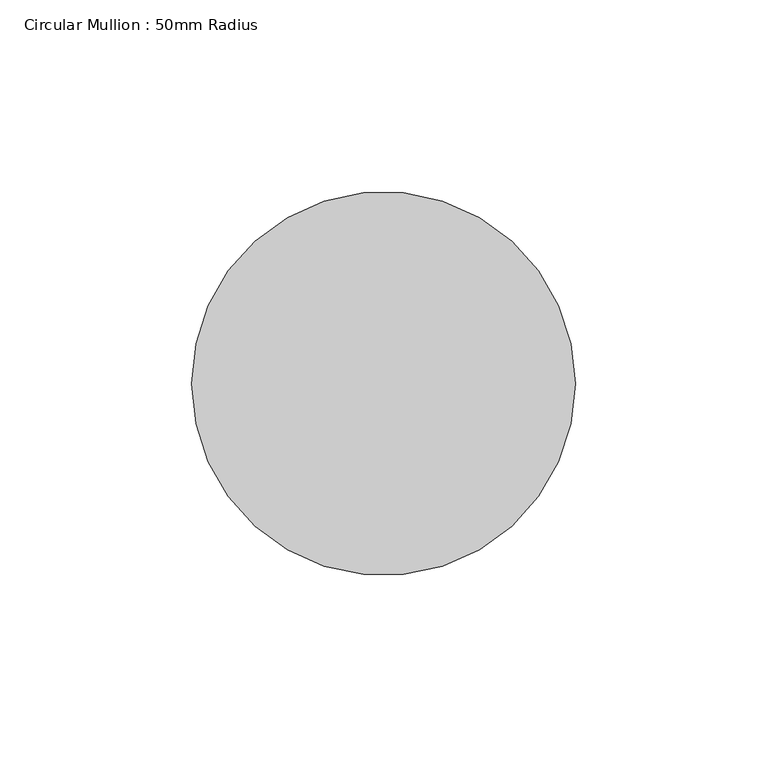
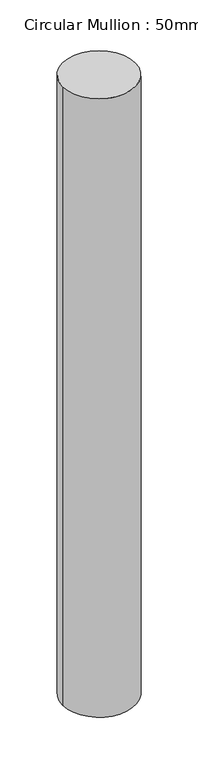
"""IFC4 building model written with IfcOpenShell, lengths in millimetres: member geometry, Circular Mullion : 50mm Radius."""

from ifc_helpers import new_model, si_unit, point, frame, origin, origin_2d, place, context, project, spatial, circle_curve, trimmed, segment, composite_curve, outline, extrude, source, transform, mapped, element, save


def circular_mullion_50mm_radius_7659f404(model_context):
    return source(origin(), model_context, "Body", "SweptSolid", [
        extrude(outline(composite_curve([segment(trimmed(circle_curve(origin_2d(), 50.0), [point((50.0, 0.0))], [point((-50.0, 0.0))], False, "CARTESIAN"), True, "CONTINUOUS"), segment(trimmed(circle_curve(origin_2d(), 50.0), [point((-50.0, 0.0))], [point((50.0, 0.0))], False, "CARTESIAN"), True, "CONTINUOUS")], self_intersect=False)), frame((0.0, 0.0, -900.5440201), z_axis=(0.0, 0.0, 1.0), x_axis=(1.0, 0.0, 0.0)), (0.0, 0.0, 1.0), 900.5440201),
    ])


if __name__ == "__main__":
    model = new_model("IFC4")
    model_context = context("Model", 3, world=origin())
    ifc_project = project(units=[si_unit("LENGTHUNIT", "METRE", prefix="MILLI")], contexts=[model_context])
    site = spatial("IfcSite", under=ifc_project)
    building = spatial("IfcBuilding", under=site)
    placement = place(None, origin())
    circular_mullion_50mm_radius_shape = circular_mullion_50mm_radius_7659f404(model_context)
    element("IfcMember", 1, ObjectType="Circular Mullion : 50mm Radius", at=placement, inside=building, context=model_context, shape_type="MappedRepresentation", body=[
        mapped(circular_mullion_50mm_radius_shape, transform((0.0, 0.0, 0.0), x_axis=(1.0, 0.0, 0.0), y_axis=(0.0, 1.0, 0.0), z_axis=(0.0, 0.0, 1.0))),
    ])
    save(model, "model.ifc")

# Revit data of these elements
# Type "Circular Mullion : 50mm Radius"
#   built-in parameter 1007350 = 0.164042 (stored number, unit not read)
# Element 1 (IfcMember, "Circular Mullion : 50mm Radius")
#   Materials on its faces: "Aluminium"
# Materials
#   "Aluminium": class "Metal", colour RGB 247 247 247, transparency 0, Description = "Aluminium 6061", Cost = 0
